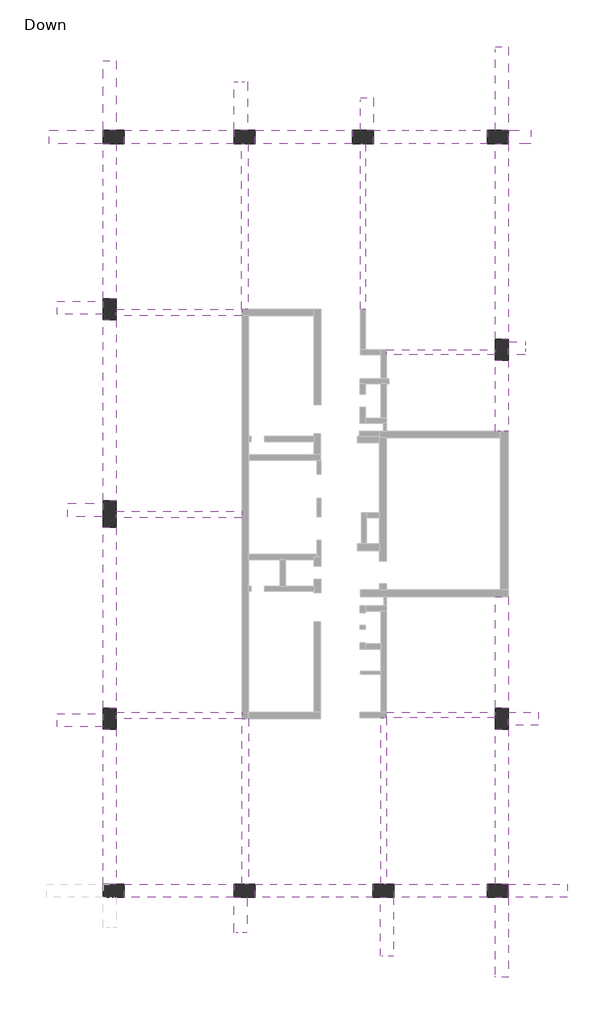
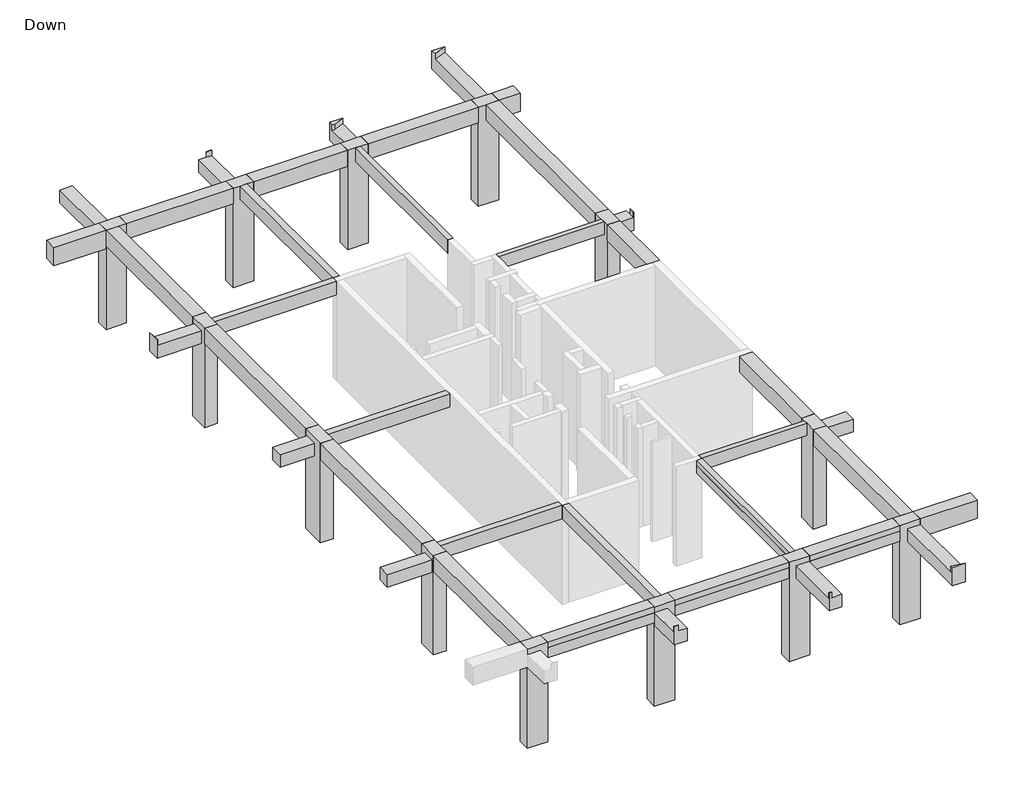
# One storey, part 2 of 2: 38 beams, 13 columns.
"""IFC4 building model written with IfcOpenShell, lengths in millimetres."""

from ifc_helpers import new_model, si_unit, frame, origin, place, context, project, spatial, polyline, outline, extrude, faceted_brep, element, save

model = new_model("IFC4")

# Units and contexts
model_context = context("Model", 3, world=origin())
ifc_project = project(units=[si_unit("LENGTHUNIT", "METRE", prefix="MILLI")], contexts=[model_context])

# Site, building, storey
site = spatial("IfcSite", under=ifc_project)
building = spatial("IfcBuilding", under=site)
storey = spatial("IfcBuildingStorey", under=building, Name="Down", Elevation=0.0)

# Beams
placement = place(None, origin())
element("IfcBeam", 1, ObjectType="Concrete Rectengular Beam : 20/50", at=placement, inside=storey, context=model_context, shape_type="Brep", body=[
    faceted_brep([(5886.2445731, 13812.7962372, 4125.0), (5886.2445731, 14012.7962372, 4125.0), (1734.6005416, 14012.7962372, 4125.0), (1734.6005416, 13812.7962372, 4125.0), (5886.2445731, 13812.7962372, 3625.0), (5886.2445731, 13812.7962372, 3895.0), (1734.6005416, 13812.7962372, 3895.0), (1734.6005416, 13812.7962372, 3625.0), (5886.2445731, 14012.7962372, 3625.0), (1734.6005416, 14012.7962372, 3625.0), (5886.2445731, 14012.7962372, 3895.0)], [[[0, 1, 2, 3]], [[4, 5, 0, 3, 6, 7]], [[8, 4, 7, 9]], [[1, 10, 8, 9, 2]], [[1, 0, 5, 4, 8, 10]], [[3, 2, 9, 7, 6]]]),
])
element("IfcBeam", 2, ObjectType="Concrete Rectengular Beam : 20/50", at=placement, inside=storey, context=model_context, shape_type="Brep", body=[
    faceted_brep([(5886.2445731, 6.0759332, 4125.0), (5886.2445731, 206.0759332, 4125.0), (1741.4745301, 206.0759332, 4125.0), (1741.4745301, 6.0759332, 4125.0), (5886.2445731, 6.0759332, 3625.0), (5886.2445731, 6.0759332, 3895.0), (1741.4745301, 6.0759332, 3895.0), (1741.4745301, 6.0759332, 3625.0), (5886.2445731, 206.0759332, 3625.0), (1741.4745301, 206.0759332, 3625.0), (5886.2445731, 206.0759332, 3895.0), (1741.4745301, 206.0759332, 3895.0)], [[[0, 1, 2, 3]], [[4, 5, 0, 3, 6, 7]], [[8, 4, 7, 9]], [[1, 10, 8, 9, 11, 2]], [[1, 0, 5, 4, 8, 10]], [[3, 2, 11, 9, 7, 6]]]),
])
element("IfcBeam", 3, ObjectType="Concrete Rectengular Beam : 20/55", at=placement, inside=storey, context=model_context, shape_type="Brep", body=[
    faceted_brep([(945.9739967, 21858.4827803, 4125.0), (745.9739967, 21858.4827803, 4125.0), (745.9739967, 15552.7962372, 4125.0), (945.9739967, 15552.7962372, 4125.0), (945.9739967, 21858.4827803, 3575.0), (945.9739967, 21858.4827803, 3895.0), (945.9739967, 15552.7962372, 3575.0), (745.9739967, 21858.4827803, 3575.0), (745.9739967, 15552.7962372, 3575.0), (745.9739967, 21858.4827803, 3895.0), (745.9739967, 15552.7962372, 3895.0)], [[[0, 1, 2, 3]], [[4, 5, 0, 3, 6]], [[7, 4, 6, 8]], [[2, 1, 9, 7, 8, 10]], [[0, 5, 4, 7, 9, 1]], [[3, 2, 10, 8, 6]]]),
])
element("IfcBeam", 4, ObjectType="Concrete Rectengular Beam : 20/55", at=placement, inside=storey, context=model_context, shape_type="Brep", body=[
    faceted_brep([(1741.4745301, -6329.9837689, 4125.0), (1741.4745301, 6.0759332, 4125.0), (1541.8129739, 6.0759332, 4125.0), (1541.8129739, -6329.9837689, 4125.0), (1541.4745301, 6.0759332, 3575.0), (1541.4745301, -6329.9837689, 3575.0), (1541.4745301, -6329.9837689, 3895.0), (1541.4745301, 6.0759332, 3895.0), (1741.4745301, -6329.9837689, 3575.0), (1741.4745301, 6.0759332, 3575.0), (1741.4745301, -6329.9837689, 3895.0), (1741.4745301, 6.0759332, 3895.0), (1541.8129739, -6329.9837689, 3895.0), (1541.8129739, 6.0759332, 3895.0)], [[[0, 1, 2, 3]], [[4, 5, 6, 7]], [[8, 5, 4, 9]], [[0, 10, 8, 9, 11, 1]], [[8, 10, 0, 3, 12, 6, 5]], [[12, 13, 7, 6]], [[13, 12, 3, 2]], [[9, 4, 7, 13, 2, 1, 11]]]),
])
element("IfcBeam", 5, ObjectType="Concrete Rectengular Beam : 25/55", at=placement, inside=storey, context=model_context, shape_type="Brep", body=[
    faceted_brep([(-3760.0513475, -6329.9837689, 4125.0), (-3510.0513475, -6329.9837689, 4125.0), (-3510.0513475, -34.8235665, 4125.0), (-3760.0513475, -34.8235665, 4125.0), (-3760.0513475, -6329.9837689, 3575.0), (-3760.0513475, -6329.9837689, 3895.0), (-3760.0513475, -34.8235665, 3895.0), (-3760.0513475, -34.8235665, 3575.0), (-3510.0513475, -6329.9837689, 3575.0), (-3510.0513475, -34.8235665, 3575.0), (-3510.0513475, -6329.9837689, 3895.0), (-3510.0513475, -34.8235665, 3895.0)], [[[0, 1, 2, 3]], [[4, 5, 0, 3, 6, 7]], [[8, 4, 7, 9]], [[2, 1, 10, 8, 9, 11]], [[0, 5, 4, 8, 10, 1]], [[3, 2, 11, 9, 7, 6]]]),
])
element("IfcBeam", 6, ObjectType="Concrete Rectengular Beam : 25/55", at=placement, inside=storey, context=model_context, shape_type="Brep", body=[
    faceted_brep([(-8554.7039512, 215.1764335, 4125.0), (-8554.7039512, -34.8235665, 4125.0), (-3760.0513475, -34.8235665, 4125.0), (-3760.0513475, 215.1764335, 4125.0), (-8554.7039512, 215.1764335, 3575.0), (-8554.7039512, 215.1764335, 3895.0), (-3760.0513475, 215.1764335, 3895.0), (-3760.0513475, 215.1764335, 3575.0), (-8554.7039512, -34.8235665, 3575.0), (-3760.0513475, -34.8235665, 3575.0), (-8554.7039512, -34.8235665, 3895.0), (-3760.0513475, -34.8235665, 3895.0)], [[[0, 1, 2, 3]], [[4, 5, 0, 3, 6, 7]], [[8, 4, 7, 9]], [[1, 10, 8, 9, 11, 2]], [[8, 10, 1, 0, 5, 4]], [[3, 2, 11, 9, 7, 6]]]),
])
element("IfcBeam", 7, ObjectType="Concrete Rectengular Beam : 25/55", at=placement, inside=storey, context=model_context, shape_type="Brep", body=[
    faceted_brep([(-8554.7039512, 7860.6259096, 4125.0), (-8554.7039512, 7610.6259096, 4125.0), (-3760.0513475, 7610.6259096, 4125.0), (-3760.0513475, 7860.6259096, 4125.0), (-8554.7039512, 7610.6259096, 3895.0), (-8554.7039512, 7610.6259096, 3575.0), (-3760.0513475, 7610.6259096, 3575.0), (-3760.0513475, 7610.6259096, 3895.0), (-8554.7039512, 7860.6259096, 3575.0), (-3760.0513475, 7860.6259096, 3575.0), (-8554.7039512, 7860.6259096, 3895.0), (-3760.0513475, 7860.6259096, 3895.0)], [[[0, 1, 2, 3]], [[1, 4, 5, 6, 7, 2]], [[5, 8, 9, 6]], [[8, 10, 0, 3, 11, 9]], [[5, 4, 1, 0, 10, 8]], [[3, 2, 7, 6, 9, 11]]]),
])
element("IfcBeam", 8, ObjectType="Concrete Rectengular Beam : 25/55", at=placement, inside=storey, context=model_context, shape_type="Brep", body=[
    faceted_brep([(-8554.7039512, 15556.1764947, 4125.0), (-8554.7039512, 15306.1764947, 4125.0), (-3760.0513475, 15306.1764947, 4125.0), (-3760.0513475, 15556.1764947, 4125.0), (-3779.0260033, 15556.1764947, 4125.0), (-8554.7039512, 15556.1764947, 3575.0), (-8554.7039512, 15556.1764947, 3895.0), (-3760.0513475, 15556.1764947, 3575.0), (-3779.0260033, 15556.1764947, 3575.0), (-8554.7039512, 15306.1764947, 3575.0), (-3760.0513475, 15306.1764947, 3575.0), (-8554.7039512, 15306.1764947, 3895.0), (-3760.0513475, 15306.1764947, 3895.0)], [[[0, 1, 2, 3, 4]], [[5, 6, 0, 4, 3, 7, 8]], [[9, 5, 8, 7, 10]], [[1, 11, 9, 10, 12, 2]], [[9, 11, 1, 0, 6, 5]], [[3, 2, 12, 10, 7]]]),
])
element("IfcBeam", 9, ObjectType="Concrete Rectengular Beam : 25/55", at=placement, inside=storey, context=model_context, shape_type="Brep", body=[
    faceted_brep([(-3529.0260033, 21858.4827803, 4125.0), (-3779.0260033, 21858.4827803, 4125.0), (-3779.0260033, 15556.1764947, 4125.0), (-3760.0513475, 15556.1764947, 4125.0), (-3529.0260033, 15556.1764947, 4125.0), (-3529.0260033, 21858.4827803, 3575.0), (-3529.0260033, 21858.4827803, 3895.0), (-3529.0260033, 15556.1764947, 3895.0), (-3529.0260033, 15556.1764947, 3575.0), (-3779.0260033, 21858.4827803, 3575.0), (-3760.0513475, 15556.1764947, 3575.0), (-3779.0260033, 15556.1764947, 3575.0), (-3779.0260033, 21858.4827803, 3895.0), (-3779.0260033, 15556.1764947, 3895.0)], [[[0, 1, 2, 3, 4]], [[5, 6, 0, 4, 7, 8]], [[9, 5, 8, 10, 11]], [[1, 12, 9, 11, 13, 2]], [[1, 0, 6, 5, 9, 12]], [[4, 3, 2, 13, 11, 10, 8, 7]]]),
])
element("IfcBeam", 10, ObjectType="Concrete Rectengular Beam : 50/75", at=placement, inside=storey, context=model_context, shape_type="Brep", body=[
    faceted_brep([(-11104.7039512, 21858.4827803, 4125.0), (-11104.7039512, 22358.4827803, 4125.0), (-11104.7039512, 22358.4827803, 3375.0), (-11104.7039512, 21858.4827803, 3375.0), (-9054.7039512, 21858.4827803, 4125.0), (-9054.7039512, 22358.4827803, 4125.0), (-9054.7039512, 22358.4827803, 3475.0), (-9054.0260033, 22358.4827803, 3475.0), (-9054.0260033, 22358.4827803, 3375.0), (-9054.7039512, 22358.4827803, 3375.0), (-9054.0260033, 21858.4827803, 3375.0), (-9054.0260033, 21858.4827803, 3475.0), (-9054.7039512, 21858.4827803, 3475.0), (-9054.7039512, 21858.4827803, 3895.0)], [[[0, 1, 2, 3]], [[1, 0, 4, 5]], [[2, 1, 5, 6, 7, 8, 9]], [[3, 2, 9, 8, 10]], [[0, 3, 10, 11, 12, 13, 4]], [[10, 8, 7, 11]], [[6, 12, 11, 7]], [[12, 6, 5, 4, 13]]]),
])
element("IfcBeam", 11, ObjectType="Concrete Rectengular Beam : 50/75", at=placement, inside=storey, context=model_context, shape_type="Brep", body=[
    faceted_brep([(-8554.7039512, 25008.4827803, 3375.0), (-9054.7039512, 25008.4827803, 3375.0), (-9054.7039512, 25008.4827803, 3895.0), (-8554.7039512, 25008.4827803, 3895.0), (-8554.7039512, 22358.4827803, 3375.0), (-8554.7039512, 22358.4827803, 3895.0), (-9054.0260033, 22358.4827803, 3375.0), (-9054.7039512, 22358.4827803, 3375.0), (-9054.7039512, 22358.4827803, 3895.0)], [[[0, 1, 2, 3]], [[4, 0, 3, 5]], [[1, 0, 4, 6, 7]], [[1, 7, 8, 2]], [[7, 6, 4, 5, 8]], [[3, 2, 8, 5]]]),
])
element("IfcBeam", 12, ObjectType="Concrete Rectengular Beam : 50/75", at=placement, inside=storey, context=model_context, shape_type="Brep", body=[
    faceted_brep([(-3554.0260033, 24208.4827803, 4125.0), (-3554.0260033, 24208.4827803, 3375.0), (-4054.0260033, 24208.4827803, 3375.0), (-4054.0260033, 24208.4827803, 3895.0), (-3764.1506551, 24208.4827803, 3895.0), (-3764.1506551, 24208.4827803, 4125.0), (-3554.0260033, 24173.3589408, 4125.0), (-3554.0260033, 24173.3589408, 3895.0), (-3554.0260033, 22358.4827803, 3895.0), (-3554.0260033, 22358.4827803, 3375.0), (-4054.0260033, 22358.4827803, 3375.0), (-4054.0260033, 22358.4827803, 3895.0)], [[[0, 1, 2, 3, 4, 5]], [[0, 5, 6]], [[1, 0, 6, 7, 8, 9]], [[2, 1, 9, 10]], [[2, 10, 11, 3]], [[10, 9, 8, 11]], [[7, 4, 3, 11, 8]], [[4, 7, 6, 5]]]),
])
element("IfcBeam", 13, ObjectType="Concrete Rectengular Beam : 50/75", at=placement, inside=storey, context=model_context, shape_type="Brep", body=[
    faceted_brep([(745.9739967, 23608.4827803, 4125.0), (1245.9739967, 23608.4827803, 4125.0), (1245.9739967, 23608.4827803, 3375.0), (745.9739967, 23608.4827803, 3375.0), (745.9739967, 23454.583164, 4125.0), (840.503122, 23438.7819441, 4125.0), (1245.9739967, 23591.5033567, 4125.0), (1245.9739967, 23591.5033567, 3895.0), (1245.9739967, 22358.4827803, 3895.0), (1245.9739967, 22358.4827803, 3375.0), (745.9739967, 22358.4827803, 3375.0), (745.9739967, 22358.4827803, 3895.0), (745.9739967, 23454.583164, 3895.0), (840.503122, 23438.7819441, 3895.0)], [[[0, 1, 2, 3]], [[1, 0, 4, 5, 6]], [[2, 1, 6, 7, 8, 9]], [[3, 2, 9, 10]], [[0, 3, 10, 11, 12, 4]], [[10, 9, 8, 11]], [[13, 12, 11, 8, 7]], [[5, 13, 7, 6]], [[13, 5, 4, 12]]]),
])
element("IfcBeam", 14, ObjectType="Concrete Rectengular Beam : 50/75", at=placement, inside=storey, context=model_context, shape_type="Brep", body=[
    faceted_brep([(5885.9739967, 25548.4827803, 4125.0), (6385.9739967, 25548.4827803, 4125.0), (6385.9739967, 25548.4827803, 3375.0), (5885.9739967, 25548.4827803, 3375.0), (5885.9739967, 25339.1685989, 4125.0), (6385.9739967, 25527.4945948, 4125.0), (6385.9739967, 25527.4945948, 3895.0), (6385.9739967, 22358.4827803, 3895.0), (6385.9739967, 22358.4827803, 3375.0), (5885.9739967, 22358.4827803, 3375.0), (5885.9739967, 22358.4827803, 3895.0), (5885.9739967, 25339.1685989, 3895.0)], [[[0, 1, 2, 3]], [[1, 0, 4, 5]], [[2, 1, 5, 6, 7, 8]], [[3, 2, 8, 9]], [[0, 3, 9, 10, 11, 4]], [[9, 8, 7, 10]], [[6, 11, 10, 7]], [[11, 6, 5, 4]]]),
])
element("IfcBeam", 15, ObjectType="Concrete Rectengular Beam : 50/75", at=placement, inside=storey, context=model_context, shape_type="Brep", body=[
    faceted_brep([(-10804.7039512, 15356.2782734, 4125.0), (-10804.7039512, 15856.2782734, 4125.0), (-10804.7039512, 15856.2782734, 3375.0), (-10804.7039512, 15356.2782734, 3375.0), (-10772.4180283, 15356.2782734, 4125.0), (-10797.9698179, 15856.2782734, 4125.0), (-10797.9698179, 15856.2782734, 3895.0), (-9054.7039512, 15856.2782734, 3895.0), (-9054.7039512, 15856.2782734, 3375.0), (-9054.7039512, 15356.2782734, 3375.0), (-9054.7039512, 15356.2782734, 3895.0), (-10772.4180283, 15356.2782734, 3895.0)], [[[0, 1, 2, 3]], [[1, 0, 4, 5]], [[2, 1, 5, 6, 7, 8]], [[3, 2, 8, 9]], [[0, 3, 9, 10, 11, 4]], [[9, 8, 7, 10]], [[6, 11, 10, 7]], [[11, 6, 5, 4]]]),
])
element("IfcBeam", 16, ObjectType="Concrete Rectengular Beam : 50/75", at=placement, inside=storey, context=model_context, shape_type="Brep", body=[
    faceted_brep([(-10404.7039512, 8160.8120649, 3375.0), (-10404.7039512, 7660.8120649, 3375.0), (-10404.7039512, 7660.8120649, 3895.0), (-10404.7039512, 7691.6468948, 3895.0), (-10404.7039512, 8160.8120649, 3895.0), (-9054.7039512, 8160.8120649, 3375.0), (-9054.7039512, 8160.8120649, 3895.0), (-9054.7039512, 7660.8120649, 3375.0), (-9054.7039512, 7660.8120649, 3895.0)], [[[0, 1, 2, 3, 4]], [[5, 0, 4, 6]], [[1, 0, 5, 7]], [[1, 7, 8, 2]], [[7, 5, 6, 8]], [[4, 3, 2, 8, 6]]]),
])
element("IfcBeam", 17, ObjectType="Concrete Rectengular Beam : 50/75", at=placement, inside=storey, context=model_context, shape_type="SweptSolid", body=[
    extrude(outline(polyline([(-10804.7039512, -334.7552972), (-10804.7039512, 165.2447028), (-9054.7039512, 165.2447028), (-9054.7039512, -334.7552972), (-10804.7039512, -334.7552972)])), frame((0.0, 0.0, 3375.0), z_axis=(0.0, 0.0, 1.0), x_axis=(1.0, 0.0, 0.0)), (0.0, 0.0, 1.0), 520.0),
])
element("IfcBeam", 18, ObjectType="Concrete Rectengular Beam : 50/75", at=placement, inside=storey, context=model_context, shape_type="Brep", body=[
    faceted_brep([(-4059.9850878, -8179.9837689, 4125.0), (-4059.9850878, -8179.9837689, 3375.0), (-3559.9850878, -8179.9837689, 3375.0), (-3559.9850878, -8179.9837689, 3895.0), (-3902.9638337, -8179.9837689, 3895.0), (-3902.9638337, -8179.9837689, 4125.0), (-4059.9850878, -8154.3832223, 4125.0), (-4059.9850878, -8154.3832223, 3895.0), (-4059.9850878, -6829.9837689, 3895.0), (-4059.9850878, -6829.9837689, 3375.0), (-3559.9850878, -6829.9837689, 3375.0), (-3559.9850878, -6829.9837689, 3895.0)], [[[0, 1, 2, 3, 4, 5]], [[0, 5, 6]], [[1, 0, 6, 7, 8, 9]], [[2, 1, 9, 10]], [[2, 10, 11, 3]], [[10, 9, 8, 11]], [[7, 4, 3, 11, 8]], [[4, 7, 6, 5]]]),
])
element("IfcBeam", 19, ObjectType="Concrete Rectengular Beam : 50/75", at=placement, inside=storey, context=model_context, shape_type="Brep", body=[
    faceted_brep([(1509.6005863, -9079.9837689, 4125.0), (1509.6005863, -9079.9837689, 3375.0), (2009.6005863, -9079.9837689, 3375.0), (2009.6005863, -9079.9837689, 3895.0), (1617.196753, -9079.9837689, 3895.0), (1617.196753, -9079.9837689, 4125.0), (1509.6005863, -9062.441426, 4125.0), (1509.6005863, -9062.441426, 3895.0), (1509.6005863, -6829.9837689, 3895.0), (1509.6005863, -6829.9837689, 3375.0), (2009.6005863, -6829.9837689, 3375.0), (2009.6005863, -6829.9837689, 3895.0)], [[[0, 1, 2, 3, 4, 5]], [[0, 5, 6]], [[1, 0, 6, 7, 8, 9]], [[2, 1, 9, 10]], [[2, 10, 11, 3]], [[10, 9, 8, 11]], [[7, 4, 3, 11, 8]], [[4, 7, 6, 5]]]),
])
element("IfcBeam", 20, ObjectType="Concrete Rectengular Beam : 50/75", at=placement, inside=storey, context=model_context, shape_type="Brep", body=[
    faceted_brep([(6386.2445731, -9879.9837689, 4125.0), (5886.2445731, -9879.9837689, 4125.0), (5886.2445731, -9879.9837689, 3375.0), (6386.2445731, -9879.9837689, 3375.0), (6386.2445731, -9857.5232935, 4125.0), (5886.2445731, -9776.0039259, 4125.0), (5886.2445731, -9776.0039259, 3895.0), (5886.2445731, -6829.9837689, 3895.0), (5886.2445731, -6829.9837689, 3475.0), (5886.2445731, -6829.9837689, 3375.0), (6385.9739967, -6829.9837689, 3375.0), (6385.9739967, -6329.9837689, 3375.0), (6386.2445731, -6329.9837689, 3375.0), (6386.2445731, -6829.9837689, 3375.0), (6386.2445731, -6329.9837689, 3475.0), (6386.2445731, -6829.9837689, 3475.0), (6386.2445731, -6829.9837689, 3895.0), (6386.2445731, -9857.5232935, 3895.0), (6385.9739967, -6829.9837689, 3475.0), (6385.9739967, -6329.9837689, 3475.0), (6385.9739967, -6829.9837689, 3895.0)], [[[0, 1, 2, 3]], [[1, 0, 4, 5]], [[2, 1, 5, 6, 7, 8, 9]], [[3, 2, 9, 10, 11, 12, 13]], [[0, 3, 13, 12, 14, 15, 16, 17, 4]], [[11, 10, 18, 19]], [[10, 9, 8, 7, 20, 16, 15, 18]], [[12, 11, 19, 14]], [[6, 17, 16, 20, 7]], [[17, 6, 5, 4]], [[18, 15, 14, 19]]]),
])
element("IfcBeam", 21, ObjectType="Concrete Rectengular Beam : 50/75", at=placement, inside=storey, context=model_context, shape_type="Brep", body=[
    faceted_brep([(8636.2445731, -6329.9837689, 4125.0), (8636.2445731, -6829.9837689, 4125.0), (8636.2445731, -6829.9837689, 3375.0), (8636.2445731, -6329.9837689, 3375.0), (6386.2445731, -6329.9837689, 4125.0), (6386.2445731, -6829.8142121, 4125.0), (6386.2445731, -6829.9837689, 4125.0), (6386.2445731, -6829.9837689, 3895.0), (6386.2445731, -6829.9837689, 3475.0), (6386.2445731, -6829.9837689, 3375.0), (6386.2445731, -6329.9837689, 3375.0), (6386.2445731, -6329.9837689, 3475.0), (6386.2445731, -6329.9837689, 3895.0)], [[[0, 1, 2, 3]], [[1, 0, 4, 5, 6]], [[2, 1, 6, 7, 8, 9]], [[3, 2, 9, 10]], [[0, 3, 10, 11, 12, 4]], [[6, 5, 4, 12, 11, 10, 9, 8, 7]]]),
])
element("IfcBeam", 22, ObjectType="Concrete Rectengular Beam : 50/75", at=placement, inside=storey, context=model_context, shape_type="SweptSolid", body=[
    extrude(outline(polyline([(7536.2445731, 222.1859334), (7536.2445731, -277.8140666), (6386.2445731, -277.8140666), (6386.2445731, 222.1859334), (7536.2445731, 222.1859334)])), frame((0.0, 0.0, 3375.0), z_axis=(0.0, 0.0, 1.0), x_axis=(1.0, 0.0, 0.0)), (0.0, 0.0, 1.0), 520.0),
])
element("IfcBeam", 23, ObjectType="Concrete Rectengular Beam : 50/75", at=placement, inside=storey, context=model_context, shape_type="Brep", body=[
    faceted_brep([(7036.2445731, 13812.897882, 4125.0), (7036.2445731, 13812.897882, 3375.0), (7036.2445731, 14312.897882, 3375.0), (7036.2445731, 14312.897882, 3895.0), (7036.2445731, 14045.149647, 3895.0), (7036.2445731, 14045.149647, 4125.0), (7030.5099098, 13821.115472, 4125.0), (7030.2995619, 13812.897882, 4125.0), (7030.2995619, 13812.897882, 3895.0), (6386.2445731, 13812.897882, 3895.0), (6386.2445731, 13812.897882, 3375.0), (6386.2445731, 14312.897882, 3375.0), (6386.2445731, 14312.897882, 3895.0), (7030.5099098, 13821.115472, 3895.0)], [[[0, 1, 2, 3, 4, 5]], [[0, 5, 6, 7]], [[1, 0, 7, 8, 9, 10]], [[2, 1, 10, 11]], [[2, 11, 12, 3]], [[11, 10, 9, 12]], [[13, 4, 3, 12, 9, 8]], [[6, 13, 8, 7]], [[13, 6, 5, 4]]]),
])
element("IfcBeam", 24, ObjectType="Concrete Rectengular Beam : 50/75", at=placement, inside=storey, context=model_context, shape_type="Brep", body=[
    faceted_brep([(7236.2445731, 22358.4827803, 4125.0), (7236.2445731, 21858.4827803, 4125.0), (7236.2445731, 21858.4827803, 3375.0), (7236.2445731, 22358.4827803, 3375.0), (6385.9739967, 22358.4827803, 4125.0), (6385.9739967, 22108.4827803, 4125.0), (6386.2445731, 22108.4827803, 4125.0), (6386.2445731, 21858.4827803, 4125.0), (6386.2445731, 21858.4827803, 3895.0), (6386.2445731, 21858.4827803, 3475.0), (6385.9739967, 21858.4827803, 3475.0), (6385.9739967, 21858.4827803, 3375.0), (6385.9739967, 22358.4827803, 3375.0), (6385.9739967, 22108.4827803, 3475.0), (6386.2445731, 22108.4827803, 3475.0)], [[[0, 1, 2, 3]], [[1, 0, 4, 5, 6, 7]], [[2, 1, 7, 8, 9, 10, 11]], [[3, 2, 11, 12]], [[0, 3, 12, 4]], [[4, 12, 11, 10, 13, 5]], [[6, 14, 9, 8, 7]], [[9, 14, 13, 10]], [[14, 6, 5, 13]]]),
])
element("IfcBeam", 25, ObjectType="Concrete Rectengular Beam : 65/50", at=placement, inside=storey, context=model_context, shape_type="SweptSolid", body=[
    extrude(outline(polyline([(-4054.0260033, 22358.4827803), (-4054.0260033, 21858.4827803), (-8254.0260033, 21858.4827803), (-8254.0260033, 22358.4827803), (-4054.0260033, 22358.4827803)])), frame((0.0, 0.0, 3475.0), z_axis=(0.0, 0.0, 1.0), x_axis=(1.0, 0.0, 0.0)), (0.0, 0.0, 1.0), 650.0),
])
element("IfcBeam", 26, ObjectType="Concrete Rectengular Beam : 65/50", at=placement, inside=storey, context=model_context, shape_type="SweptSolid", body=[
    extrude(outline(polyline([(445.9739967, 22358.4827803), (445.9739967, 21858.4827803), (-3254.0260033, 21858.4827803), (-3254.0260033, 22358.4827803), (445.9739967, 22358.4827803)])), frame((0.0, 0.0, 3475.0), z_axis=(0.0, 0.0, 1.0), x_axis=(1.0, 0.0, 0.0)), (0.0, 0.0, 1.0), 650.0),
])
element("IfcBeam", 27, ObjectType="Concrete Rectengular Beam : 65/50", at=placement, inside=storey, context=model_context, shape_type="SweptSolid", body=[
    extrude(outline(polyline([(5585.9739967, 22358.4827803), (5585.9739967, 21858.4827803), (1245.9739967, 21858.4827803), (1245.9739967, 22358.4827803), (5585.9739967, 22358.4827803)])), frame((0.0, 0.0, 3475.0), z_axis=(0.0, 0.0, 1.0), x_axis=(1.0, 0.0, 0.0)), (0.0, 0.0, 1.0), 650.0),
])
element("IfcBeam", 28, ObjectType="Concrete Rectengular Beam : 65/50", at=placement, inside=storey, context=model_context, shape_type="Brep", body=[
    faceted_brep([(6386.2445731, 22108.4827803, 4125.0), (6385.9739967, 22108.4827803, 4125.0), (6385.9739967, 21858.4827803, 4125.0), (6386.2445731, 21858.4827803, 4125.0), (6386.2445731, 22108.4827803, 3475.0), (6386.2445731, 21858.4827803, 3895.0), (6386.2445731, 14412.6609936, 3895.0), (6386.2445731, 14412.6609936, 3475.0), (6386.2445731, 21858.4827803, 3475.0), (5886.2445731, 14412.6609936, 3475.0), (5886.2445731, 21858.4827803, 3475.0), (6385.9739967, 21858.4827803, 3475.0), (6385.9739967, 22108.4827803, 3475.0), (5886.2445731, 21858.4827803, 4125.0), (5886.2445731, 21858.4827803, 3895.0), (5886.2445731, 14412.6609936, 4125.0), (6385.5385444, 21858.4827803, 4125.0), (6385.5385444, 21858.4827803, 3895.0), (6385.9739967, 21858.4827803, 3895.0), (6385.5385444, 14412.6609936, 3895.0), (6385.5385444, 14412.6609936, 4125.0)], [[[0, 1, 2, 3]], [[4, 0, 3, 5, 6, 7, 8]], [[7, 9, 10, 11, 12, 4, 8]], [[13, 14, 10, 9, 15]], [[0, 4, 12, 1]], [[10, 14, 13, 16, 17, 18, 11]], [[2, 1, 12, 11, 18]], [[9, 7, 6, 19, 20, 15]], [[5, 18, 17, 19, 6]], [[19, 17, 16, 20]], [[18, 5, 3, 2]], [[13, 15, 20, 16]]]),
])
element("IfcBeam", 29, ObjectType="Concrete Rectengular Beam : 65/50", at=placement, inside=storey, context=model_context, shape_type="Brep", body=[
    faceted_brep([(5886.2445731, 13612.6609936, 4125.0), (5886.2445731, 10911.592205, 4125.0), (6086.2445731, 10911.592205, 4125.0), (6385.5385444, 10911.592205, 4125.0), (6385.5385444, 13612.6609936, 4125.0), (5886.2445731, 13612.6609936, 3475.0), (5886.2445731, 10911.592205, 3475.0), (5886.2445731, 10911.592205, 3895.0), (6386.2445731, 13612.6609936, 3475.0), (6386.2445731, 10911.592205, 3475.0), (6386.2445731, 13612.6609936, 3895.0), (6386.2445731, 10911.592205, 3895.0), (6385.5385444, 13612.6609936, 3895.0), (6385.5385444, 10911.592205, 3895.0)], [[[0, 1, 2, 3, 4]], [[0, 5, 6, 7, 1]], [[5, 8, 9, 6]], [[9, 8, 10, 11]], [[5, 0, 4, 12, 10, 8]], [[1, 7, 6, 9, 11, 13, 3, 2]], [[12, 13, 11, 10]], [[13, 12, 4, 3]]]),
])
element("IfcBeam", 30, ObjectType="Concrete Rectengular Beam : 65/50", at=placement, inside=storey, context=model_context, shape_type="Brep", body=[
    faceted_brep([(5886.2445731, 4616.7541606, 4125.0), (5886.2445731, 372.1859334, 4125.0), (6385.5385444, 372.1859334, 4125.0), (6385.5385444, 4616.7541606, 4125.0), (6386.2445731, 372.1859334, 3475.0), (6386.2445731, 4616.7541606, 3475.0), (6386.2445731, 4616.7541606, 3895.0), (6386.2445731, 372.1859334, 3895.0), (5886.2445731, 372.1859334, 3475.0), (5886.2445731, 4616.7541606, 3475.0), (5886.2445731, 4616.7541606, 3895.0), (6385.5385444, 372.1859334, 3895.0), (6385.5385444, 4616.7541606, 3895.0)], [[[0, 1, 2, 3]], [[4, 5, 6, 7]], [[4, 8, 9, 5]], [[8, 1, 0, 10, 9]], [[8, 4, 7, 11, 2, 1]], [[5, 9, 10, 0, 3, 12, 6]], [[12, 11, 7, 6]], [[11, 12, 3, 2]]]),
])
element("IfcBeam", 31, ObjectType="Concrete Rectengular Beam : 65/50", at=placement, inside=storey, context=model_context, shape_type="Brep", body=[
    faceted_brep([(6385.9739967, -6329.9837689, 4125.0), (6385.9739967, -6829.8142121, 4125.0), (6386.2445731, -6829.8142121, 4125.0), (6386.2445731, -6329.9837689, 4125.0), (5886.2445731, -6329.9837689, 3475.0), (5886.2445731, -6329.9837689, 3895.0), (5886.2445731, -6329.9837689, 4125.0), (5886.2445731, -427.8140666, 4125.0), (5886.2445731, -427.8140666, 3475.0), (6385.9739967, -6329.9837689, 3475.0), (6386.2445731, -427.8140666, 3475.0), (6386.2445731, -6329.9837689, 3475.0), (6386.2445731, -6829.9837689, 3475.0), (6385.9739967, -6829.9837689, 3475.0), (6386.2445731, -427.8140666, 3895.0), (6386.2445731, -6329.9837689, 3895.0), (6386.2445731, -6829.8142121, 3895.0), (6386.2445731, -6829.9837689, 3895.0), (6385.9739967, -6329.9837689, 3895.0), (6385.5385444, -6329.9837689, 3895.0), (6385.5385444, -6329.9837689, 4125.0), (6385.9739967, -6829.9837689, 3895.0), (6385.9739967, -6829.8142121, 3895.0), (6385.5385444, -427.8140666, 4125.0), (6385.5385444, -427.8140666, 3895.0)], [[[0, 1, 2, 3]], [[4, 5, 6, 7, 8]], [[9, 4, 8, 10, 11, 12, 13]], [[12, 11, 10, 14, 15, 3, 2, 16, 17]], [[6, 5, 4, 9, 18, 19, 20]], [[9, 13, 21, 22, 1, 0, 18]], [[8, 7, 23, 24, 14, 10]], [[13, 12, 17, 21]], [[16, 22, 21, 17]], [[22, 16, 2, 1]], [[24, 19, 18, 15, 14]], [[15, 18, 0, 3]], [[19, 24, 23, 20]], [[7, 6, 20, 23]]]),
])
element("IfcBeam", 32, ObjectType="Concrete Rectengular Beam : 65/50", at=placement, inside=storey, context=model_context, shape_type="SweptSolid", body=[
    extrude(outline(polyline([(-6329.9837689, 4125.0), (-6329.9837689, 3475.0), (-6829.9837689, 3475.0), (-6829.9837689, 3895.0), (-6829.8142121, 3895.0), (-6829.8142121, 4125.0), (-6329.9837689, 4125.0)])), frame((2034.4987629, 0.0, 0.0), z_axis=(1.0, 0.0, 0.0), x_axis=(0.0, 1.0, 0.0)), (0.0, 0.0, 1.0), 3551.4752338),
])
element("IfcBeam", 33, ObjectType="Concrete Rectengular Beam : 65/50", at=placement, inside=storey, context=model_context, shape_type="SweptSolid", body=[
    extrude(outline(polyline([(-6329.9837689, 4125.0), (-6329.9837689, 3475.0), (-6829.9837689, 3475.0), (-6829.9837689, 3895.0), (-6829.8142121, 3895.0), (-6829.8142121, 4125.0), (-6329.9837689, 4125.0)])), frame((-3260.1545107, 0.0, 0.0), z_axis=(1.0, 0.0, 0.0), x_axis=(0.0, 1.0, 0.0)), (0.0, 0.0, 1.0), 4494.6532735),
])
element("IfcBeam", 34, ObjectType="Concrete Rectengular Beam : 65/50", at=placement, inside=storey, context=model_context, shape_type="SweptSolid", body=[
    extrude(outline(polyline([(-6329.9837689, 4125.0), (-6329.9837689, 3475.0), (-6829.9837689, 3475.0), (-6829.9837689, 3895.0), (-6829.8142121, 3895.0), (-6829.8142121, 4125.0), (-6329.9837689, 4125.0)])), frame((-8254.7039512, 0.0, 0.0), z_axis=(1.0, 0.0, 0.0), x_axis=(0.0, 1.0, 0.0)), (0.0, 0.0, 1.0), 4194.5494405),
])
element("IfcBeam", 35, ObjectType="Concrete Rectengular Beam : 65/50", at=placement, inside=storey, context=model_context, shape_type="Brep", body=[
    faceted_brep([(-9054.7039512, -6329.9837689, 4125.0), (-8554.7039512, -6329.9837689, 4125.0), (-8554.7039512, -427.8140666, 4125.0), (-9054.7039512, -427.8140666, 4125.0), (-9054.7039512, -6329.8142121, 4125.0), (-9054.7039512, -6329.9837689, 3475.0), (-9054.7039512, -427.8140666, 3475.0), (-9054.7039512, -6329.8142121, 3475.0), (-8554.7039512, -6329.9837689, 3475.0), (-8554.7039512, -427.8140666, 3475.0), (-8554.7039512, -6329.8142121, 3475.0), (-8554.7039512, -6329.9837689, 3895.0)], [[[0, 1, 2, 3, 4]], [[5, 0, 4, 3, 6, 7]], [[8, 5, 7, 6, 9, 10]], [[1, 11, 8, 10, 9, 2]], [[1, 0, 5, 8, 11]], [[3, 2, 9, 6]]]),
    faceted_brep([(-8804.7039512, -6832.2071205, 3475.0), (-8655.7238806, -6832.2071205, 3475.0), (-8655.7238806, -6832.2071205, 3895.0), (-8804.7039512, -6832.2071205, 3895.0), (-8655.7238806, -6829.9837689, 3475.0), (-8655.7238806, -6829.9837689, 3895.0), (-8804.7039512, -6829.9837689, 3475.0), (-8804.7039512, -6829.9837689, 3895.0)], [[[0, 1, 2, 3]], [[1, 4, 5, 2]], [[6, 0, 3, 7]], [[4, 6, 7, 5]], [[1, 0, 6, 4]], [[3, 2, 5, 7]]]),
])
element("IfcBeam", 36, ObjectType="Concrete Rectengular Beam : 65/50", at=placement, inside=storey, context=model_context, shape_type="SweptSolid", body=[
    extrude(outline(polyline([(-8554.7039512, 372.1859334), (-9054.7039512, 372.1859334), (-9054.7039512, 7260.8455297), (-8554.7039512, 7260.8455297), (-8554.7039512, 372.1859334)])), frame((0.0, 0.0, 3475.0), z_axis=(0.0, 0.0, 1.0), x_axis=(1.0, 0.0, 0.0)), (0.0, 0.0, 1.0), 650.0),
])
element("IfcBeam", 37, ObjectType="Concrete Rectengular Beam : 65/50", at=placement, inside=storey, context=model_context, shape_type="SweptSolid", body=[
    extrude(outline(polyline([(-8554.7039512, 8260.8455297), (-9054.7039512, 8260.8455297), (-9054.7039512, 15152.1859334), (-8554.7039512, 15152.1859334), (-8554.7039512, 8260.8455297)])), frame((0.0, 0.0, 3475.0), z_axis=(0.0, 0.0, 1.0), x_axis=(1.0, 0.0, 0.0)), (0.0, 0.0, 1.0), 650.0),
])
element("IfcBeam", 38, ObjectType="Concrete Rectengular Beam : 65/50", at=placement, inside=storey, context=model_context, shape_type="Brep", body=[
    faceted_brep([(-9054.7039512, 15952.1859334, 4125.0), (-8554.7039512, 15952.1859334, 4125.0), (-8554.7039512, 21858.4827803, 4125.0), (-9054.7039512, 21858.4827803, 4125.0), (-8554.7039512, 15952.1859334, 3475.0), (-8554.7039512, 21858.4827803, 3475.0), (-8554.7039512, 21858.4827803, 3895.0), (-9054.7039512, 15952.1859334, 3475.0), (-9054.7039512, 21858.4827803, 3475.0), (-9054.7039512, 21858.4827803, 3895.0)], [[[0, 1, 2, 3]], [[1, 4, 5, 6, 2]], [[4, 7, 8, 5]], [[7, 0, 3, 9, 8]], [[2, 6, 5, 8, 9, 3]], [[1, 0, 7, 4]]]),
])

# Columns
element("IfcColumn", 39, ObjectType="Concrete Rectengular Column : 50/100", at=placement, inside=storey, context=model_context, shape_type="Brep", body=[
    faceted_brep([(-8554.7039512, 8260.8455297, 0.0), (-8554.7039512, 7260.8455297, 0.0), (-9054.7039512, 7260.8455297, 0.0), (-9054.7039512, 8260.8455297, 0.0), (-8554.7039512, 8260.8455297, 4125.0), (-8554.7039512, 7860.6259096, 4125.0), (-8554.7039512, 7610.6259096, 4125.0), (-8554.7039512, 7260.8455297, 4125.0), (-9054.7039512, 7260.8455297, 4125.0), (-9054.7039512, 8260.8455297, 4125.0)], [[[0, 1, 2, 3]], [[4, 5, 6, 7, 1, 0]], [[7, 8, 2, 1]], [[8, 9, 3, 2]], [[9, 4, 0, 3]], [[4, 9, 8, 7, 6, 5]]]),
])
element("IfcColumn", 40, ObjectType="Concrete Rectengular Column : 50/80", at=placement, inside=storey, context=model_context, shape_type="Brep", body=[
    faceted_brep([(5585.9739967, 22358.4827803, 0.0), (6385.9739967, 22358.4827803, 0.0), (6385.9739967, 21858.4827803, 0.0), (5585.9739967, 21858.4827803, 0.0), (5585.9739967, 22358.4827803, 4125.0), (6385.9739967, 22358.4827803, 4125.0), (6385.9739967, 21858.4827803, 4125.0), (6385.5385444, 21858.4827803, 4125.0), (5886.2445731, 21858.4827803, 4125.0), (5585.9739967, 21858.4827803, 4125.0)], [[[0, 1, 2, 3]], [[4, 5, 1, 0]], [[5, 6, 2, 1]], [[6, 7, 8, 9, 3, 2]], [[9, 4, 0, 3]], [[4, 9, 8, 7, 6, 5]]]),
])
element("IfcColumn", 41, ObjectType="Concrete Rectengular Column : 50/80", at=placement, inside=storey, context=model_context, shape_type="Brep", body=[
    faceted_brep([(445.9739967, 22358.4827803, 0.0), (1245.9739967, 22358.4827803, 0.0), (1245.9739967, 21858.4827803, 0.0), (445.9739967, 21858.4827803, 0.0), (445.9739967, 22358.4827803, 4125.0), (1245.9739967, 22358.4827803, 4125.0), (1245.9739967, 21858.4827803, 4125.0), (945.9739967, 21858.4827803, 4125.0), (745.9739967, 21858.4827803, 4125.0), (445.9739967, 21858.4827803, 4125.0)], [[[0, 1, 2, 3]], [[4, 5, 1, 0]], [[5, 6, 2, 1]], [[6, 7, 8, 9, 3, 2]], [[9, 4, 0, 3]], [[4, 9, 8, 7, 6, 5]]]),
])
element("IfcColumn", 42, ObjectType="Concrete Rectengular Column : 50/80", at=placement, inside=storey, context=model_context, shape_type="Brep", body=[
    faceted_brep([(-4054.0260033, 22358.4827803, 0.0), (-3254.0260033, 22358.4827803, 0.0), (-3254.0260033, 21858.4827803, 0.0), (-4054.0260033, 21858.4827803, 0.0), (-4054.0260033, 22358.4827803, 4125.0), (-3254.0260033, 22358.4827803, 4125.0), (-3254.0260033, 21858.4827803, 4125.0), (-3529.0260033, 21858.4827803, 4125.0), (-3779.0260033, 21858.4827803, 4125.0), (-4054.0260033, 21858.4827803, 4125.0)], [[[0, 1, 2, 3]], [[4, 5, 1, 0]], [[5, 6, 2, 1]], [[6, 7, 8, 9, 3, 2]], [[9, 4, 0, 3]], [[4, 9, 8, 7, 6, 5]]]),
])
element("IfcColumn", 43, ObjectType="Concrete Rectengular Column : 50/80", at=placement, inside=storey, context=model_context, shape_type="Brep", body=[
    faceted_brep([(-9054.0260033, 22358.4827803, 0.0), (-8254.0260033, 22358.4827803, 0.0), (-8254.0260033, 21858.4827803, 0.0), (-9054.0260033, 21858.4827803, 0.0), (-9054.0260033, 22358.4827803, 4125.0), (-8254.0260033, 22358.4827803, 4125.0), (-8254.0260033, 21858.4827803, 4125.0), (-8554.7039512, 21858.4827803, 4125.0), (-9054.0260033, 21858.4827803, 4125.0)], [[[0, 1, 2, 3]], [[4, 5, 1, 0]], [[5, 6, 2, 1]], [[6, 7, 8, 3, 2]], [[8, 4, 0, 3]], [[4, 8, 7, 6, 5]]]),
])
element("IfcColumn", 44, ObjectType="Concrete Rectengular Column : 50/80", at=placement, inside=storey, context=model_context, shape_type="Brep", body=[
    faceted_brep([(5585.9739967, -6329.9837689, 0.0), (6385.9739967, -6329.9837689, 0.0), (6385.9739967, -6829.9837689, 0.0), (5585.9739967, -6829.9837689, 0.0), (5585.9739967, -6329.9837689, 4125.0), (5886.2445731, -6329.9837689, 4125.0), (6385.5385444, -6329.9837689, 4125.0), (6385.9739967, -6329.9837689, 4125.0), (6385.9739967, -6829.9837689, 4125.0), (6385.9739967, -6829.9837689, 3895.0), (5585.9739967, -6829.9837689, 4125.0), (5585.9739967, -6829.9837689, 3895.0)], [[[0, 1, 2, 3]], [[4, 5, 6, 7, 1, 0]], [[7, 8, 9, 2, 1]], [[8, 10, 11, 3, 2, 9]], [[10, 4, 0, 3, 11]], [[4, 10, 8, 7, 6, 5]]]),
])
element("IfcColumn", 45, ObjectType="Concrete Rectengular Column : 50/80", at=placement, inside=storey, context=model_context, shape_type="Brep", body=[
    faceted_brep([(1234.4987629, -6329.9837689, 0.0), (2034.4987629, -6329.9837689, 0.0), (2034.4987629, -6829.9837689, 0.0), (1234.4987629, -6829.9837689, 0.0), (1234.4987629, -6329.9837689, 4125.0), (1541.8129739, -6329.9837689, 4125.0), (1741.4745301, -6329.9837689, 4125.0), (2034.4987629, -6329.9837689, 4125.0), (2034.4987629, -6829.9837689, 4125.0), (2034.4987629, -6829.9837689, 3895.0), (1234.4987629, -6829.9837689, 4125.0), (1234.4987629, -6829.9837689, 3895.0)], [[[0, 1, 2, 3]], [[4, 5, 6, 7, 1, 0]], [[7, 8, 9, 2, 1]], [[8, 10, 11, 3, 2, 9]], [[10, 4, 0, 3, 11]], [[4, 10, 8, 7, 6, 5]]]),
])
element("IfcColumn", 46, ObjectType="Concrete Rectengular Column : 50/80", at=placement, inside=storey, context=model_context, shape_type="Brep", body=[
    faceted_brep([(-4060.1545107, -6329.9837689, 0.0), (-3260.1545107, -6329.9837689, 0.0), (-3260.1545107, -6829.9837689, 0.0), (-4060.1545107, -6829.9837689, 0.0), (-4060.1545107, -6329.9837689, 4125.0), (-3760.0513475, -6329.9837689, 4125.0), (-3510.0513475, -6329.9837689, 4125.0), (-3260.1545107, -6329.9837689, 4125.0), (-3260.1545107, -6829.9837689, 4125.0), (-3260.1545107, -6829.9837689, 3895.0), (-4060.1545107, -6829.9837689, 4125.0), (-4060.1545107, -6829.9837689, 3895.0)], [[[0, 1, 2, 3]], [[4, 5, 6, 7, 1, 0]], [[7, 8, 9, 2, 1]], [[8, 10, 11, 3, 2, 9]], [[10, 4, 0, 3, 11]], [[4, 10, 8, 7, 6, 5]]]),
])
element("IfcColumn", 47, ObjectType="Concrete Rectengular Column : 50/80", at=placement, inside=storey, context=model_context, shape_type="Brep", body=[
    faceted_brep([(-8254.7039512, -6829.9837689, 0.0), (-9054.7039512, -6829.9837689, 0.0), (-9054.7039512, -6329.9837689, 0.0), (-8254.7039512, -6329.9837689, 0.0), (-8254.7039512, -6829.9837689, 4125.0), (-9054.7039512, -6829.9837689, 4125.0), (-9054.7039512, -6829.9837689, 3895.0), (-8254.7039512, -6829.9837689, 3895.0), (-9054.7039512, -6329.9837689, 4125.0), (-8554.7039512, -6329.9837689, 4125.0), (-8254.7039512, -6329.9837689, 4125.0)], [[[0, 1, 2, 3]], [[4, 5, 6, 1, 0, 7]], [[5, 8, 2, 1, 6]], [[8, 9, 10, 3, 2]], [[10, 4, 7, 0, 3]], [[4, 10, 9, 8, 5]]]),
])
element("IfcColumn", 48, ObjectType="Concrete Rectengular Column : 50/80", at=placement, inside=storey, context=model_context, shape_type="Brep", body=[
    faceted_brep([(-8554.7039512, 372.1859334, 0.0), (-8554.7039512, -427.8140666, 0.0), (-9054.7039512, -427.8140666, 0.0), (-9054.7039512, 372.1859334, 0.0), (-8554.7039512, 372.1859334, 4125.0), (-8554.7039512, 215.1764335, 4125.0), (-8554.7039512, -34.8235665, 4125.0), (-8554.7039512, -427.8140666, 4125.0), (-9054.7039512, -427.8140666, 4125.0), (-9054.7039512, 372.1859334, 4125.0)], [[[0, 1, 2, 3]], [[4, 5, 6, 7, 1, 0]], [[7, 8, 2, 1]], [[8, 9, 3, 2]], [[9, 4, 0, 3]], [[4, 9, 8, 7, 6, 5]]]),
])
element("IfcColumn", 49, ObjectType="Concrete Rectengular Column : 50/80", at=placement, inside=storey, context=model_context, shape_type="Brep", body=[
    faceted_brep([(-8554.7039512, 15952.1859334, 0.0), (-8554.7039512, 15152.1859334, 0.0), (-9054.7039512, 15152.1859334, 0.0), (-9054.7039512, 15952.1859334, 0.0), (-8554.7039512, 15952.1859334, 4125.0), (-8554.7039512, 15556.1764947, 4125.0), (-8554.7039512, 15306.1764947, 4125.0), (-8554.7039512, 15152.1859334, 4125.0), (-9054.7039512, 15152.1859334, 4125.0), (-9054.7039512, 15952.1859334, 4125.0)], [[[0, 1, 2, 3]], [[4, 5, 6, 7, 1, 0]], [[7, 8, 2, 1]], [[8, 9, 3, 2]], [[9, 4, 0, 3]], [[4, 9, 8, 7, 6, 5]]]),
])
element("IfcColumn", 50, ObjectType="Concrete Rectengular Column : 50/80", at=placement, inside=storey, context=model_context, shape_type="Brep", body=[
    faceted_brep([(6386.2445731, 14412.6609936, 0.0), (6386.2445731, 13612.6609936, 0.0), (5886.2445731, 13612.6609936, 0.0), (5886.2445731, 14412.6609936, 0.0), (6386.2445731, 14412.6609936, 4125.0), (6386.2445731, 13612.6609936, 4125.0), (6386.2445731, 13612.6609936, 3895.0), (6386.2445731, 14412.6609936, 3895.0), (5886.2445731, 13612.6609936, 4125.0), (5886.2445731, 13812.7962372, 4125.0), (5886.2445731, 14012.7962372, 4125.0), (5886.2445731, 14412.6609936, 4125.0)], [[[0, 1, 2, 3]], [[4, 5, 6, 1, 0, 7]], [[5, 8, 2, 1, 6]], [[8, 9, 10, 11, 3, 2]], [[11, 4, 7, 0, 3]], [[4, 11, 10, 9, 8, 5]]]),
])
element("IfcColumn", 51, ObjectType="Concrete Rectengular Column : 50/80", at=placement, inside=storey, context=model_context, shape_type="Brep", body=[
    faceted_brep([(6386.2445731, 372.1859334, 0.0), (6386.2445731, -427.8140666, 0.0), (5886.2445731, -427.8140666, 0.0), (5886.2445731, 372.1859334, 0.0), (6386.2445731, 372.1859334, 4125.0), (6386.2445731, -427.8140666, 4125.0), (6386.2445731, -427.8140666, 3895.0), (6386.2445731, 372.1859334, 3895.0), (5886.2445731, -427.8140666, 4125.0), (5886.2445731, 6.0759332, 4125.0), (5886.2445731, 206.0759332, 4125.0), (5886.2445731, 372.1859334, 4125.0)], [[[0, 1, 2, 3]], [[4, 5, 6, 1, 0, 7]], [[5, 8, 2, 1, 6]], [[8, 9, 10, 11, 3, 2]], [[11, 4, 7, 0, 3]], [[4, 11, 10, 9, 8, 5]]]),
])

save(model, "model.ifc")

# Revit data of these elements
# Type "Concrete Rectengular Beam : 20/50"
#   Length [instance default] = 152.4 cm
#   b = 20 cm
#   h = 50 cm
#   Structural Material [instance default] = Concrete
#   Assembly Code = ""
# Type "Concrete Rectengular Beam : 20/55"
#   Length [instance default] = 152.4 cm
#   b = 20 cm
#   h = 55 cm
#   Structural Material [instance default] = Concrete
#   Assembly Code = ""
# Type "Concrete Rectengular Beam : 25/55"
#   Length [instance default] = 152.4 cm
#   b = 25 cm
#   h = 55 cm
#   Structural Material [instance default] = Concrete
#   Assembly Code = ""
# Type "Concrete Rectengular Beam : 50/75"
#   Length [instance default] = 152.4 cm
#   b = 50 cm
#   h = 75 cm
#   Structural Material [instance default] = Concrete
#   Assembly Code = ""
# Type "Concrete Rectengular Beam : 65/50"
#   Length [instance default] = 152.4 cm
#   b = 50 cm
#   h = 65 cm
#   Structural Material [instance default] = Concrete
#   Assembly Code = ""
# Type "Concrete Rectengular Column : 50/100"
#   b = 50 cm
#   h = 100 cm
#   Structural Material [instance default] = Concrete
# Type "Concrete Rectengular Column : 50/80"
#   b = 50 cm
#   h = 80 cm
#   Structural Material [instance default] = Concrete
# Element 1 (IfcBeam, "Concrete Rectengular Beam : 20/50")
#   Comments = ""
#   Mark = "B1"
#   SOFiSTiK_AMG_Comments = ""
#   SOFiSTiK_AMG_Scheduled = yes
#   SOFiSTiK_AMG_Adjusted = yes
#   Structural Material = Concrete
#   Phase Created = New Construction
#   Materials on its faces: "Concrete"
# Element 2 (IfcBeam, "Concrete Rectengular Beam : 20/50")
#   Comments = ""
#   Mark = "B2"
#   SOFiSTiK_AMG_Comments = ""
#   SOFiSTiK_AMG_Scheduled = yes
#   SOFiSTiK_AMG_Adjusted = yes
#   Structural Material = Concrete
#   Phase Created = New Construction
#   Materials on its faces: "Concrete"
# Element 3 (IfcBeam, "Concrete Rectengular Beam : 20/55")
#   Comments = ""
#   Mark = "B4"
#   SOFiSTiK_AMG_Comments = ""
#   SOFiSTiK_AMG_Scheduled = yes
#   SOFiSTiK_AMG_Adjusted = yes
#   Structural Material = Concrete
#   Phase Created = New Construction
#   Materials on its faces: "Concrete"
# Element 4 (IfcBeam, "Concrete Rectengular Beam : 20/55")
#   Comments = ""
#   Mark = "B5"
#   SOFiSTiK_AMG_Comments = ""
#   SOFiSTiK_AMG_Scheduled = yes
#   SOFiSTiK_AMG_Adjusted = yes
#   Structural Material = Concrete
#   Phase Created = New Construction
#   Materials on its faces: "Concrete"
# Element 5 (IfcBeam, "Concrete Rectengular Beam : 25/55")
#   Comments = ""
#   Mark = "B6"
#   SOFiSTiK_AMG_Comments = ""
#   SOFiSTiK_AMG_Scheduled = yes
#   SOFiSTiK_AMG_Adjusted = yes
#   Structural Material = Concrete
#   Phase Created = New Construction
#   Materials on its faces: "Concrete"
# Element 6 (IfcBeam, "Concrete Rectengular Beam : 25/55")
#   Comments = ""
#   Mark = "B7"
#   SOFiSTiK_AMG_Comments = ""
#   SOFiSTiK_AMG_Scheduled = yes
#   SOFiSTiK_AMG_Adjusted = yes
#   Structural Material = Concrete
#   Phase Created = New Construction
#   Materials on its faces: "Concrete"
# Element 7 (IfcBeam, "Concrete Rectengular Beam : 25/55")
#   Comments = ""
#   Mark = "B8"
#   SOFiSTiK_AMG_Comments = ""
#   SOFiSTiK_AMG_Scheduled = yes
#   SOFiSTiK_AMG_Adjusted = yes
#   Structural Material = Concrete
#   Phase Created = New Construction
#   Materials on its faces: "Concrete"
# Element 8 (IfcBeam, "Concrete Rectengular Beam : 25/55")
#   Comments = ""
#   Mark = "B9"
#   SOFiSTiK_AMG_Comments = ""
#   SOFiSTiK_AMG_Scheduled = yes
#   SOFiSTiK_AMG_Adjusted = yes
#   Structural Material = Concrete
#   Phase Created = New Construction
#   Materials on its faces: "Concrete"
# Element 9 (IfcBeam, "Concrete Rectengular Beam : 25/55")
#   Comments = ""
#   Mark = "B10"
#   SOFiSTiK_AMG_Comments = ""
#   SOFiSTiK_AMG_Scheduled = yes
#   SOFiSTiK_AMG_Adjusted = yes
#   Structural Material = Concrete
#   Phase Created = New Construction
#   Materials on its faces: "Concrete"
# Element 10 (IfcBeam, "Concrete Rectengular Beam : 50/75")
#   Comments = ""
#   Mark = "B11"
#   SOFiSTiK_AMG_Comments = ""
#   SOFiSTiK_AMG_Scheduled = yes
#   SOFiSTiK_AMG_Adjusted = yes
#   Structural Material = Concrete
#   Phase Created = New Construction
#   Materials on its faces: "Concrete"
# Element 11 (IfcBeam, "Concrete Rectengular Beam : 50/75")
#   Comments = ""
#   Mark = "B12"
#   SOFiSTiK_AMG_Comments = ""
#   SOFiSTiK_AMG_Scheduled = yes
#   SOFiSTiK_AMG_Adjusted = yes
#   Structural Material = Concrete
#   Phase Created = New Construction
#   Materials on its faces: "Concrete"
# Element 12 (IfcBeam, "Concrete Rectengular Beam : 50/75")
#   Comments = ""
#   Mark = "B13"
#   SOFiSTiK_AMG_Comments = ""
#   SOFiSTiK_AMG_Scheduled = yes
#   SOFiSTiK_AMG_Adjusted = yes
#   Structural Material = Concrete
#   Phase Created = New Construction
#   Materials on its faces: "Concrete"
# Element 13 (IfcBeam, "Concrete Rectengular Beam : 50/75")
#   Comments = ""
#   Mark = "B14"
#   SOFiSTiK_AMG_Comments = ""
#   SOFiSTiK_AMG_Scheduled = yes
#   SOFiSTiK_AMG_Adjusted = yes
#   Structural Material = Concrete
#   Phase Created = New Construction
#   Materials on its faces: "Concrete"
# Element 14 (IfcBeam, "Concrete Rectengular Beam : 50/75")
#   Comments = ""
#   Mark = "B15"
#   SOFiSTiK_AMG_Comments = ""
#   SOFiSTiK_AMG_Scheduled = yes
#   SOFiSTiK_AMG_Adjusted = yes
#   Structural Material = Concrete
#   Phase Created = New Construction
#   Materials on its faces: "Concrete"
# Element 15 (IfcBeam, "Concrete Rectengular Beam : 50/75")
#   Comments = ""
#   Mark = "B16"
#   SOFiSTiK_AMG_Comments = ""
#   SOFiSTiK_AMG_Scheduled = yes
#   SOFiSTiK_AMG_Adjusted = yes
#   Structural Material = Concrete
#   Phase Created = New Construction
#   Materials on its faces: "Concrete"
# Element 16 (IfcBeam, "Concrete Rectengular Beam : 50/75")
#   Comments = ""
#   Mark = "B17"
#   SOFiSTiK_AMG_Comments = ""
#   SOFiSTiK_AMG_Scheduled = yes
#   SOFiSTiK_AMG_Adjusted = yes
#   Structural Material = Concrete
#   Phase Created = New Construction
#   Materials on its faces: "Concrete"
# Element 17 (IfcBeam, "Concrete Rectengular Beam : 50/75")
#   Comments = ""
#   Mark = "B18"
#   SOFiSTiK_AMG_Comments = ""
#   SOFiSTiK_AMG_Scheduled = yes
#   SOFiSTiK_AMG_Adjusted = yes
#   Structural Material = Concrete
#   Phase Created = New Construction
#   Materials on its faces: "Concrete"
# Element 18 (IfcBeam, "Concrete Rectengular Beam : 50/75")
#   Comments = ""
#   Mark = "B21"
#   SOFiSTiK_AMG_Comments = ""
#   SOFiSTiK_AMG_Scheduled = yes
#   SOFiSTiK_AMG_Adjusted = yes
#   Structural Material = Concrete
#   Phase Created = New Construction
#   Materials on its faces: "Concrete"
# Element 19 (IfcBeam, "Concrete Rectengular Beam : 50/75")
#   Comments = ""
#   Mark = "B22"
#   SOFiSTiK_AMG_Comments = ""
#   SOFiSTiK_AMG_Scheduled = yes
#   SOFiSTiK_AMG_Adjusted = yes
#   Structural Material = Concrete
#   Phase Created = New Construction
#   Materials on its faces: "Concrete"
# Element 20 (IfcBeam, "Concrete Rectengular Beam : 50/75")
#   Comments = ""
#   Mark = "B23"
#   SOFiSTiK_AMG_Comments = ""
#   SOFiSTiK_AMG_Scheduled = yes
#   SOFiSTiK_AMG_Adjusted = yes
#   Structural Material = Concrete
#   Phase Created = New Construction
#   Materials on its faces: "Concrete"
# Element 21 (IfcBeam, "Concrete Rectengular Beam : 50/75")
#   Comments = ""
#   Mark = "B24"
#   SOFiSTiK_AMG_Comments = ""
#   SOFiSTiK_AMG_Scheduled = yes
#   SOFiSTiK_AMG_Adjusted = yes
#   Structural Material = Concrete
#   Phase Created = New Construction
#   Materials on its faces: "Concrete"
# Element 22 (IfcBeam, "Concrete Rectengular Beam : 50/75")
#   Comments = ""
#   Mark = "B25"
#   SOFiSTiK_AMG_Comments = ""
#   SOFiSTiK_AMG_Scheduled = yes
#   SOFiSTiK_AMG_Adjusted = yes
#   Structural Material = Concrete
#   Phase Created = New Construction
#   Materials on its faces: "Concrete"
# Element 23 (IfcBeam, "Concrete Rectengular Beam : 50/75")
#   Comments = ""
#   Mark = "B26"
#   SOFiSTiK_AMG_Comments = ""
#   SOFiSTiK_AMG_Scheduled = yes
#   SOFiSTiK_AMG_Adjusted = yes
#   Structural Material = Concrete
#   Phase Created = New Construction
#   Materials on its faces: "Concrete"
# Element 24 (IfcBeam, "Concrete Rectengular Beam : 50/75")
#   Comments = ""
#   Mark = "B27"
#   SOFiSTiK_AMG_Comments = ""
#   SOFiSTiK_AMG_Scheduled = yes
#   SOFiSTiK_AMG_Adjusted = yes
#   Structural Material = Concrete
#   Phase Created = New Construction
#   Materials on its faces: "Concrete"
# Element 25 (IfcBeam, "Concrete Rectengular Beam : 65/50")
#   Comments = ""
#   Mark = "B28"
#   SOFiSTiK_AMG_Comments = ""
#   SOFiSTiK_AMG_Scheduled = yes
#   SOFiSTiK_AMG_Adjusted = yes
#   Structural Material = Concrete
#   Phase Created = New Construction
#   Materials on its faces: "Concrete"
# Element 26 (IfcBeam, "Concrete Rectengular Beam : 65/50")
#   Comments = ""
#   Mark = "B29"
#   SOFiSTiK_AMG_Comments = ""
#   SOFiSTiK_AMG_Scheduled = yes
#   SOFiSTiK_AMG_Adjusted = yes
#   Structural Material = Concrete
#   Phase Created = New Construction
#   Materials on its faces: "Concrete"
# Element 27 (IfcBeam, "Concrete Rectengular Beam : 65/50")
#   Comments = ""
#   Mark = "B30"
#   SOFiSTiK_AMG_Comments = ""
#   SOFiSTiK_AMG_Scheduled = yes
#   SOFiSTiK_AMG_Adjusted = yes
#   Structural Material = Concrete
#   Phase Created = New Construction
#   Materials on its faces: "Concrete"
# Element 28 (IfcBeam, "Concrete Rectengular Beam : 65/50")
#   Comments = ""
#   Mark = "B31"
#   SOFiSTiK_AMG_Comments = ""
#   SOFiSTiK_AMG_Scheduled = yes
#   SOFiSTiK_AMG_Adjusted = yes
#   Structural Material = Concrete
#   Phase Created = New Construction
#   Materials on its faces: "Concrete"
# Element 29 (IfcBeam, "Concrete Rectengular Beam : 65/50")
#   Comments = ""
#   Mark = "B32"
#   SOFiSTiK_AMG_Comments = ""
#   SOFiSTiK_AMG_Scheduled = yes
#   SOFiSTiK_AMG_Adjusted = yes
#   Structural Material = Concrete
#   Phase Created = New Construction
#   Materials on its faces: "Concrete"
# Element 30 (IfcBeam, "Concrete Rectengular Beam : 65/50")
#   Comments = ""
#   Mark = "B33"
#   SOFiSTiK_AMG_Comments = ""
#   SOFiSTiK_AMG_Scheduled = yes
#   SOFiSTiK_AMG_Adjusted = yes
#   Structural Material = Concrete
#   Phase Created = New Construction
#   Materials on its faces: "Concrete"
# Element 31 (IfcBeam, "Concrete Rectengular Beam : 65/50")
#   Comments = ""
#   Mark = "B34"
#   SOFiSTiK_AMG_Comments = ""
#   SOFiSTiK_AMG_Scheduled = yes
#   SOFiSTiK_AMG_Adjusted = yes
#   Structural Material = Concrete
#   Phase Created = New Construction
#   Materials on its faces: "Concrete"
# Element 32 (IfcBeam, "Concrete Rectengular Beam : 65/50")
#   Comments = ""
#   Mark = "B35"
#   SOFiSTiK_AMG_Comments = ""
#   SOFiSTiK_AMG_Scheduled = yes
#   SOFiSTiK_AMG_Adjusted = yes
#   Structural Material = Concrete
#   Phase Created = New Construction
#   Materials on its faces: "Concrete"
# Element 33 (IfcBeam, "Concrete Rectengular Beam : 65/50")
#   Comments = ""
#   Mark = "B36"
#   SOFiSTiK_AMG_Comments = ""
#   SOFiSTiK_AMG_Scheduled = yes
#   SOFiSTiK_AMG_Adjusted = yes
#   Structural Material = Concrete
#   Phase Created = New Construction
#   Materials on its faces: "Concrete"
# Element 34 (IfcBeam, "Concrete Rectengular Beam : 65/50")
#   Comments = ""
#   Mark = "B37"
#   SOFiSTiK_AMG_Comments = ""
#   SOFiSTiK_AMG_Scheduled = yes
#   SOFiSTiK_AMG_Adjusted = yes
#   Structural Material = Concrete
#   Phase Created = New Construction
#   Materials on its faces: "Concrete"
# Element 35 (IfcBeam, "Concrete Rectengular Beam : 65/50")
#   Comments = ""
#   Mark = "B38"
#   SOFiSTiK_AMG_Comments = ""
#   SOFiSTiK_AMG_Scheduled = yes
#   SOFiSTiK_AMG_Adjusted = yes
#   Structural Material = Concrete
#   Phase Created = New Construction
#   Materials on its faces: "Concrete"
# Element 36 (IfcBeam, "Concrete Rectengular Beam : 65/50")
#   Comments = ""
#   Mark = "B39"
#   SOFiSTiK_AMG_Comments = ""
#   SOFiSTiK_AMG_Scheduled = yes
#   SOFiSTiK_AMG_Adjusted = yes
#   Structural Material = Concrete
#   Phase Created = New Construction
#   Materials on its faces: "Concrete"
# Element 37 (IfcBeam, "Concrete Rectengular Beam : 65/50")
#   Comments = ""
#   Mark = "B40"
#   SOFiSTiK_AMG_Comments = ""
#   SOFiSTiK_AMG_Scheduled = yes
#   SOFiSTiK_AMG_Adjusted = yes
#   Structural Material = Concrete
#   Phase Created = New Construction
#   Materials on its faces: "Concrete"
# Element 38 (IfcBeam, "Concrete Rectengular Beam : 65/50")
#   Comments = ""
#   Mark = "B41"
#   SOFiSTiK_AMG_Comments = ""
#   SOFiSTiK_AMG_Scheduled = yes
#   SOFiSTiK_AMG_Adjusted = yes
#   Structural Material = Concrete
#   Phase Created = New Construction
#   Materials on its faces: "Concrete"
